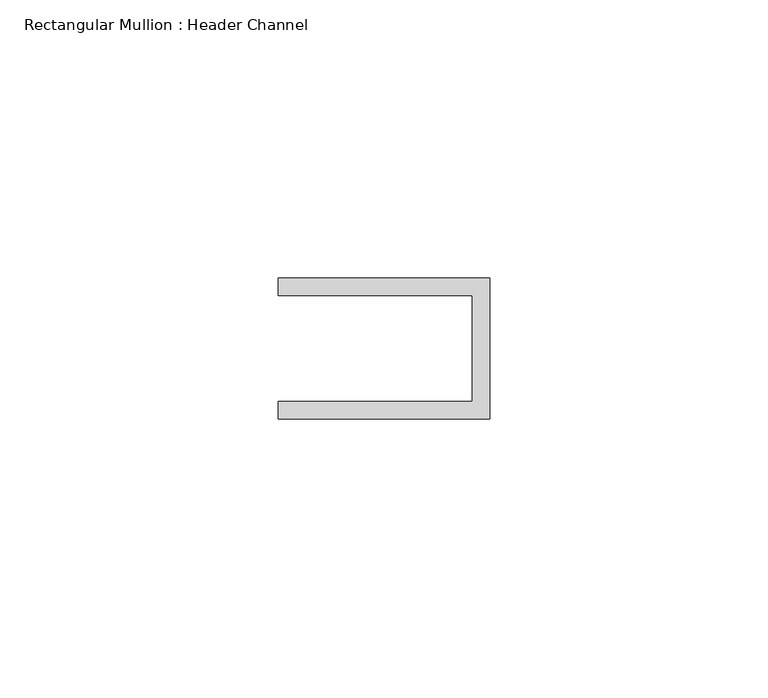
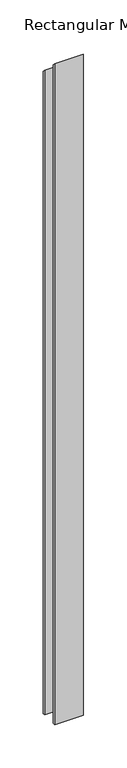
"""IFC4 building model written with IfcOpenShell, lengths in millimetres: member geometry, Rectangular Mullion : Header Channel."""

from ifc_helpers import new_model, si_unit, origin, place, context, project, spatial, faceted_brep, source, transform, mapped, element, save


def rectangular_mullion_header_channel_620b9653(model_context):
    return source(origin(), model_context, "Body", "Brep", [
        faceted_brep([(0.0, -12.7, -914.4000003), (-38.1, -12.7, -914.4000003), (-38.1, -9.525, -914.4000003), (-3.175, -9.525, -914.4000003), (-3.175, 9.525, -914.4000003), (-38.1, 9.525, -914.4000003), (-38.1, 12.7, -914.4000003), (0.0, 12.7, -914.4000003), (0.0, 12.7, -12.7), (0.0, -12.7, 12.7), (-38.1, 12.7, -12.7), (-38.1, 9.525, -9.525), (-3.175, 9.525, -9.525), (-3.175, -9.525, 9.525), (-38.1, -9.525, 9.525), (-38.1, -12.7, 12.7)], [[[0, 1, 2, 3, 4, 5, 6, 7]], [[8, 9, 0, 7]], [[10, 8, 7, 6]], [[11, 10, 6, 5]], [[12, 11, 5, 4]], [[13, 12, 4, 3]], [[14, 13, 3, 2]], [[15, 14, 2, 1]], [[9, 15, 1, 0]], [[9, 8, 10, 11, 12, 13, 14, 15]]]),
    ])


if __name__ == "__main__":
    model = new_model("IFC4")
    model_context = context("Model", 3, world=origin())
    ifc_project = project(units=[si_unit("LENGTHUNIT", "METRE", prefix="MILLI")], contexts=[model_context])
    site = spatial("IfcSite", under=ifc_project)
    building = spatial("IfcBuilding", under=site)
    placement = place(None, origin())
    rectangular_mullion_header_channel_shape = rectangular_mullion_header_channel_620b9653(model_context)
    element("IfcMember", 1, ObjectType="Rectangular Mullion : Header Channel", at=placement, inside=building, context=model_context, shape_type="MappedRepresentation", body=[
        mapped(rectangular_mullion_header_channel_shape, transform((0.0, 0.0, 0.0), x_axis=(1.0, 0.0, 0.0), y_axis=(0.0, 1.0, 0.0), z_axis=(0.0, 0.0, 1.0))),
    ])
    save(model, "model.ifc")

# Revit data of these elements
# Type "Rectangular Mullion : Header Channel"
#   built-in parameter 1007322 = 0.0833333 (stored number, unit not read)
#   built-in parameter 1007321 = -0.03125 (stored number, unit not read)
#   built-in parameter 1007320 = 0.0416667 (stored number, unit not read)
# Element 1 (IfcMember, "Rectangular Mullion : Header Channel")
#   Materials on its faces: "ALUM"
# Materials
#   "ALUM": class "Generic", colour RGB 157 157 157, transparency 0, Cost = 0
